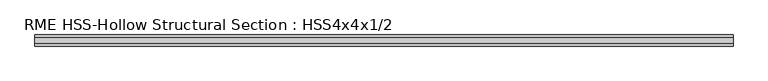
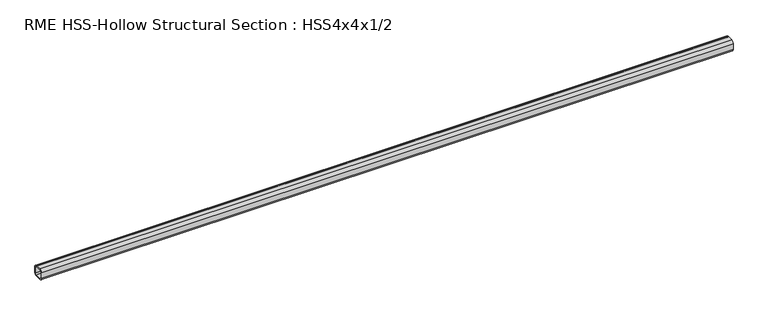
"""IFC4 building model written with IfcOpenShell, lengths in millimetres: member geometry, RME HSS-Hollow Structural Section : HSS4x4x1/2."""

from ifc_helpers import new_model, si_unit, point, frame, frame_2d, origin, place, context, project, spatial, polyline, circle_curve, trimmed, segment, composite_curve, outline, extrude, source, transform, mapped, element, save


def rme_hss_hollow_structural_section_hss4x4x1_2_1a9907fb(model_context):
    return source(origin(), model_context, "Body", "SweptSolid", [
        extrude(outline(composite_curve([segment(polyline([(50.8, 27.178), (50.8, -27.178)]), True, "CONTINUOUS"), segment(trimmed(circle_curve(frame_2d((27.178, -27.178)), 23.622), [point((50.8, -27.178))], [point((27.178, -50.8))], False, "CARTESIAN"), True, "CONTINUOUS"), segment(polyline([(27.178, -50.8), (-27.178, -50.8)]), True, "CONTINUOUS"), segment(trimmed(circle_curve(frame_2d((-27.178, -27.178)), 23.622), [point((-27.178, -50.8))], [point((-50.8, -27.178))], False, "CARTESIAN"), True, "CONTINUOUS"), segment(polyline([(-50.8, -27.178), (-50.8, 27.178)]), True, "CONTINUOUS"), segment(trimmed(circle_curve(frame_2d((-27.178, 27.178)), 23.622), [point((-50.8, 27.178))], [point((-27.178, 50.8))], False, "CARTESIAN"), True, "CONTINUOUS"), segment(polyline([(-27.178, 50.8), (27.178, 50.8)]), True, "CONTINUOUS"), segment(trimmed(circle_curve(frame_2d((27.178, 27.178)), 23.622), [point((27.178, 50.8))], [point((50.8, 27.178))], False, "CARTESIAN"), True, "CONTINUOUS")], self_intersect=False), holes=[composite_curve([segment(trimmed(circle_curve(frame_2d((-27.178, 27.178)), 11.811), [point((-27.178, 38.989))], [point((-38.989, 27.178))], True, "CARTESIAN"), True, "CONTINUOUS"), segment(polyline([(-38.989, 27.178), (-38.989, -27.178)]), True, "CONTINUOUS"), segment(trimmed(circle_curve(frame_2d((-27.178, -27.178)), 11.811), [point((-38.989, -27.178))], [point((-27.178, -38.989))], True, "CARTESIAN"), True, "CONTINUOUS"), segment(polyline([(-27.178, -38.989), (27.178, -38.989)]), True, "CONTINUOUS"), segment(trimmed(circle_curve(frame_2d((27.178, -27.178)), 11.811), [point((27.178, -38.989))], [point((38.989, -27.178))], True, "CARTESIAN"), True, "CONTINUOUS"), segment(polyline([(38.989, -27.178), (38.989, 27.178)]), True, "CONTINUOUS"), segment(trimmed(circle_curve(frame_2d((27.178, 27.178)), 11.811), [point((38.989, 27.178))], [point((27.178, 38.989))], True, "CARTESIAN"), True, "CONTINUOUS"), segment(polyline([(27.178, 38.989), (-27.178, 38.989)]), True, "CONTINUOUS")], self_intersect=False)]), frame((-3236.9281069, 0.0, 0.0), z_axis=(1.0, 0.0, 0.0), x_axis=(0.0, 1.0, 0.0)), (0.0, 0.0, 1.0), 6375.5685087),
    ])


if __name__ == "__main__":
    model = new_model("IFC4")
    model_context = context("Model", 3, world=origin())
    ifc_project = project(units=[si_unit("LENGTHUNIT", "METRE", prefix="MILLI")], contexts=[model_context])
    site = spatial("IfcSite", under=ifc_project)
    building = spatial("IfcBuilding", under=site)
    placement = place(None, origin())
    rme_hss_hollow_structural_section_hss4x4x1_2_shape = rme_hss_hollow_structural_section_hss4x4x1_2_1a9907fb(model_context)
    element("IfcMember", 1, ObjectType="RME HSS-Hollow Structural Section : HSS4x4x1/2", at=placement, inside=building, context=model_context, shape_type="MappedRepresentation", body=[
        mapped(rme_hss_hollow_structural_section_hss4x4x1_2_shape, transform((0.0, 0.0, 0.0), x_axis=(1.0, 0.0, 0.0), y_axis=(0.0, 1.0, 0.0), z_axis=(0.0, 0.0, 1.0))),
    ])
    save(model, "model.ifc")

# Revit data of these elements
# Type "RME HSS-Hollow Structural Section : HSS4x4x1/2"
#   Nominal Size = "HSS6x4"
#   Assembly Code = "B10"
#   Shape = "Square"
#   W = 21.5
#   Start Extension Calculation [instance default] = 10' - 0"
#   Start Extension [instance default] = -0' - 0 1/2"
#   End Extension Calculation [instance default] = 10' - 0"
#   End Extension [instance default] = -0' - 0 1/2"
#   Ht = 0' - 4"
#   Length [instance default] = 5' - 0"
#   b = 0' - 4"
#   kr = 0' - 0.93"
#   t = 0' - 0.465"
#   A = 0.0418056 SF
#   Structural Material [instance default] = Metal - Steel - ASTM A500 - Grade B - Rectangular and Square
# Element 1 (IfcMember, "RME HSS-Hollow Structural Section : HSS4x4x1/2")
#   Length = 22' - 11.97196"
#   Structural Material = Metal - Steel - ASTM A992
#   Materials on its faces: "Metal - Steel - ASTM A992"
# Materials
#   "Metal - Steel - ASTM A500 - Grade B - Rectangular and Square": class "Metal", colour RGB 255 128 0, transparency 0
#   "Metal - Steel - ASTM A992": class "Metal", colour RGB 255 128 0, transparency 0
